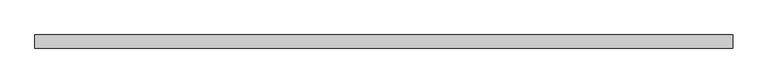
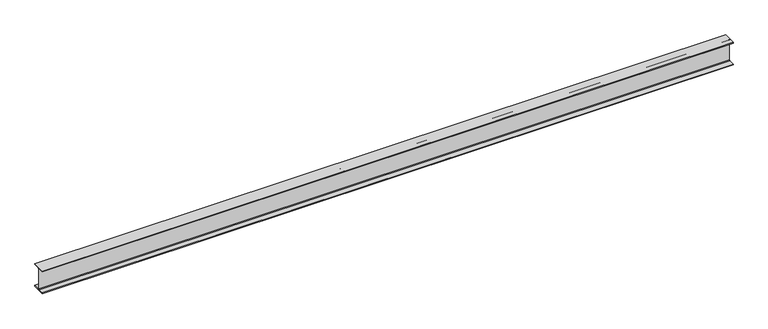
"""IFC4 building model written with IfcOpenShell, lengths in millimetres: beam geometry, Old_Steel Beam_H-KSD3502 : H_SB_ASB_H-300×300x10x15."""

from ifc_helpers import new_model, si_unit, point, frame, frame_2d, origin, place, context, project, spatial, polyline, circle_curve, trimmed, segment, composite_curve, outline, extrude, source, transform, mapped, element, save


def beam_c2b09830(model_context):
    return source(origin(), model_context, "Body", "SweptSolid", [
        extrude(outline(composite_curve([segment(polyline([(82.5, -141.5), (82.5, -151.7), (-82.5, -151.7), (-82.5, -141.5), (-11.9, -141.5)]), True, "CONTINUOUS"), segment(trimmed(circle_curve(frame_2d((-11.9, -132.6)), 8.9), [point((-11.9, -141.5))], [point((-3.0, -132.6))], True, "CARTESIAN"), True, "CONTINUOUS"), segment(polyline([(-3.0, -132.6), (-3.0, 132.6)]), True, "CONTINUOUS"), segment(trimmed(circle_curve(frame_2d((-11.9, 132.6)), 8.9), [point((-3.0, 132.6))], [point((-11.9, 141.5))], True, "CARTESIAN"), True, "CONTINUOUS"), segment(polyline([(-11.9, 141.5), (-82.5, 141.5), (-82.5, 151.7), (82.5, 151.7), (82.5, 141.5), (11.9, 141.5)]), True, "CONTINUOUS"), segment(trimmed(circle_curve(frame_2d((11.9, 132.6)), 8.9), [point((11.9, 141.5))], [point((3.0, 132.6))], True, "CARTESIAN"), True, "CONTINUOUS"), segment(polyline([(3.0, 132.6), (3.0, -132.6)]), True, "CONTINUOUS"), segment(trimmed(circle_curve(frame_2d((11.9, -132.6)), 8.9), [point((3.0, -132.6))], [point((11.9, -141.5))], True, "CARTESIAN"), True, "CONTINUOUS"), segment(polyline([(11.9, -141.5), (82.5, -141.5)]), True, "CONTINUOUS")], self_intersect=False)), frame((-4522.4440295, 0.0, 0.0), z_axis=(1.0, 0.0, 0.0), x_axis=(0.0, 1.0, 0.0)), (0.0, 0.0, 1.0), 8795.3692077),
    ])


if __name__ == "__main__":
    model = new_model("IFC4")
    model_context = context("Model", 3, world=origin())
    ifc_project = project(units=[si_unit("LENGTHUNIT", "METRE", prefix="MILLI")], contexts=[model_context])
    site = spatial("IfcSite", under=ifc_project)
    building = spatial("IfcBuilding", under=site)
    placement = place(None, origin())
    beam_shape = beam_c2b09830(model_context)
    element("IfcBeam", 1, ObjectType="Old_Steel Beam_H-KSD3502 : H_SB_ASB_H-300×300x10x15", at=placement, inside=building, context=model_context, shape_type="MappedRepresentation", body=[
        mapped(beam_shape, transform((0.0, 0.0, 0.0), x_axis=(1.0, 0.0, 0.0), y_axis=(0.0, 1.0, 0.0), z_axis=(0.0, 0.0, 1.0))),
    ])
    save(model, "model.ifc")

# Revit data of these elements
# Type "Old_Steel Beam_H-KSD3502 : H_SB_ASB_H-300×300x10x15"
#   Width = 30.0 cm
#   Web Thickness = 1.0 cm
#   Web Fillet = 1.8 cm
#   Warping Constant = 1370670.0 cm⁶
#   Torsional Moment of Inertia = 77.00 cm⁴
#   Torsional Modulus = 1.0 cm³
#   Section Area = 119.8 cm²
#   Plastic Modulus weak axis = 684.0 cm³
#   Plastic Modulus strong axis = 1500.0 cm³
#   Perimeter = 1.75 m²/m
#   Nominal Weight = 94.00 kgf/m
#   Moment of Inertia weak axis = 6750.00 cm⁴
#   Moment of Inertia strong axis = 20400.00 cm⁴
#   Height = 30.0 cm
#   Flange Thickness = 1.5 cm
#   Elastic Modulus weak axis = 450.0 cm³
#   Elastic Modulus strong axis = 1360.0 cm³
#   Centroid Vertical = 15.0 cm
#   Centroid Horizontal = 15.0 cm
#   Length [instance default] = 1.5240 m
#   Structural Material [instance default] = Steel, 45-345
#   Assembly Code = ""
# Element 1 (IfcBeam, "Old_Steel Beam_H-KSD3502 : H_SB_ASB_H-300×300x10x15")
#   Structural Material = none
# Materials
#   "Steel, 45-345": class "Metal", colour RGB 189 187 185, transparency 0, Description = "Steel 345 MPa", Cost = 0
